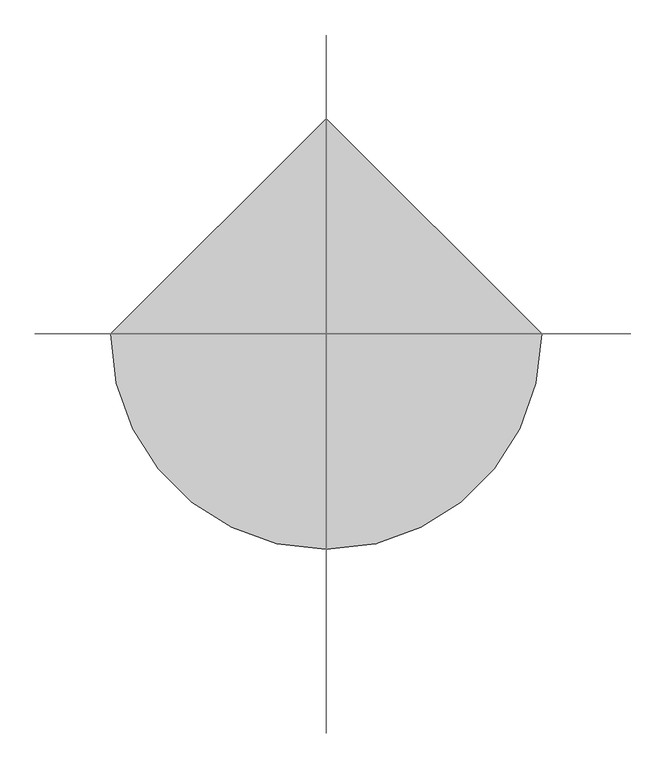
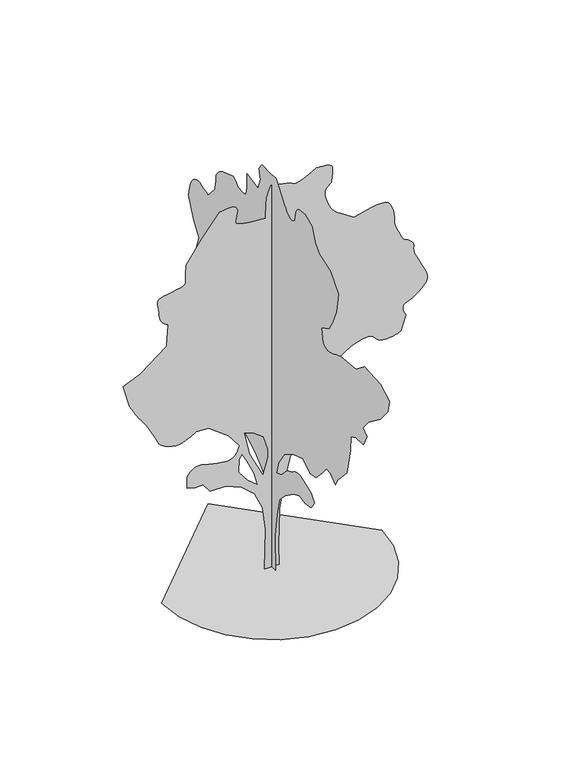
"""IFC4 building model written with IfcOpenShell, lengths in millimetres: proxy geometry, japanese flowering cherry 26172 : japanese flowering cherry 26172."""

from ifc_helpers import new_model, si_unit, origin, place, context, project, spatial, triangles, source, transform, mapped, element, save


def entourage_e499737d(model_context):
    return source(origin(), model_context, "Body", "Tessellation", [
        triangles([(-0.0028028, 75.7657196, 0.0059537), (-0.0028028, -73.2478183, 0.0059537), (-0.0028028, -59.7012251, 399.6312029), (-0.0028028, -100.3410047, 663.7914597), (-0.0028028, -147.7544623, 866.9916292), (-0.0028028, -256.1287339, 982.1375078), (-0.0028028, -418.6863261, 1097.2859299), (-0.0028028, -527.0605977, 1144.6976435), (-0.0028028, -635.434833, 1124.3775902), (-0.0028028, -750.5807842, 1144.6976435), (-0.0028028, -811.5407988, 1232.7519344), (-0.0028028, -750.5807842, 1314.0320023), (-0.0028028, -533.8347845, 1388.5377743), (-0.0028028, -514.9955638, 1387.0189716), (-0.0028028, -496.3341665, 1385.0834793), (-0.0028028, -478.0283798, 1382.3173691), (-0.0028028, -460.2559908, 1378.3091835), (-0.0028028, -443.1947865, 1372.6425236), (-0.0028028, -427.0200471, 1364.9005543), (-0.0028028, -411.9146828, 1354.6719635), (-0.0028028, -396.8067387, 1343.65345), (-0.0028028, -380.6345427, 1333.6991158), (-0.0028028, -363.5733384, 1324.6364422), (-0.0028028, -345.8009494, 1316.2824463), (-0.0028028, -327.4951627, 1308.4643188), (-0.0028028, -308.8337654, 1300.9992222), (-0.0028028, -289.994581, 1293.7118763), (-0.0028028, -188.3942419, 1185.3376774), (-0.0028028, -86.7944115, 1144.6976435), (-0.0028028, -127.4344454, 1286.9377258), (-0.0028028, -242.580869, 1456.2720119), (-0.0028028, -405.140496, 1557.8722057), (-0.0028028, -594.794799, 1618.8321476), (-0.0028028, -730.2607309, 1530.7779293), (-0.0028028, -838.6350025, 1544.3263756), (-0.0028028, -953.7809538, 1666.2439339), (-0.0028028, -1041.8351721, 1774.6181328), (-0.0028028, -1123.1126965, 1767.8439823), (-0.0028028, -1211.1669147, 1686.5663853), (-0.0028028, -1265.3528515, 1781.3922832), (-0.0028028, -1326.3127934, 1849.1240501), (-0.0028028, -1434.6871376, 1964.2723995), (-0.0028028, -1502.4187592, 2269.0726902), (-0.0028028, -1509.193055, 2431.6328259), (-0.0028028, -1604.0214237, 2472.2703163), (-0.0028028, -1753.0332584, 2485.8186172), (-0.0028028, -1813.9932003, 2614.5002975), (-0.0028028, -1739.4874283, 2675.4602394), (-0.0028028, -1841.0874767, 2797.3804138), (-0.0028028, -2071.3792339, 2973.5042564), (-0.0028028, -2220.3935394, 3149.6025192), (-0.0028028, -2247.4851997, 3291.8426743), (-0.0028028, -2078.1535297, 3386.6610146), (-0.0028028, -1766.5790886, 3400.2244308), (-0.0028028, -1610.7931034, 3278.3045471), (-0.0028028, -1312.7669632, 3244.4208595), (-0.0028028, -1272.2845505, 3228.5456657), (-0.0028028, -1232.7519344, 3213.2041603), (-0.0028028, -1195.1115721, 3198.9294502), (-0.0028028, -1160.3186377, 3186.2546425), (-0.0028028, -1129.3153702, 3175.7137161), (-0.0028028, -1103.0517843, 3167.8397781), (-0.0028028, -1082.4726625, 3163.1406464), (-0.0028028, -1064.0500225, 3162.8865921), (-0.0028028, -1044.5580437, 3166.9000099), (-0.0028028, -1025.4242552, 3173.6309944), (-0.0028028, -1008.065867, 3181.5558014), (-0.0028028, -993.907865, 3189.1248161), (-0.0028028, -984.3701477, 3194.789296), (-0.0028028, -980.8726141, 3197.024334), (-0.0028028, -947.0067307, 3359.5844696), (-0.0028028, -1089.2468857, 3434.0828293), (-0.0028028, -1156.9810507, 3542.4645859), (-0.0028028, -1231.4868954, 3718.5628487), (-0.0028028, -1272.127002, 3942.0832169), (-0.0028028, -1116.3410168, 4118.1814796), (-0.0028028, -913.1409199, 4192.7051285), (-0.0028028, -831.8608521, 4267.2034882), (-0.0028028, -770.9007648, 4429.7636238), (-0.0028028, -628.6606825, 4483.9417122), (-0.0028028, -605.4958537, 4483.8402649), (-0.0028028, -582.6891789, 4483.1542603), (-0.0028028, -560.5911455, 4481.2747238), (-0.0028028, -539.5599438, 4477.6426781), (-0.0028028, -519.9511116, 4471.5974075), (-0.0028028, -502.1202959, 4462.6310944), (-0.0028028, -486.4205638, 4450.0836044), (-0.0028028, -473.6824242, 4434.3863068), (-0.0028028, -464.1447433, 4416.5554184), (-0.0028028, -457.2740144, 4396.9467316), (-0.0028028, -452.5343691, 4375.9154572), (-0.0028028, -449.3949532, 4353.8173874), (-0.0028028, -447.3197528, 4331.0083145), (-0.0028028, -445.7805299, 4307.8434494), (-0.0028028, -434.0914178, 4294.9401672), (-0.0028028, -421.9248276, 4283.0531021), (-0.0028028, -408.8133096, 4273.1978897), (-0.0028028, -394.279422, 4266.3398781), (-0.0028028, -377.850701, 4263.5202827), (-0.0028028, -359.0495956, 4265.7303223), (-0.0028028, -337.4062583, 4273.9853416), (-0.0028028, -315.9610193, 4285.9741447), (-0.0028028, -297.7161846, 4298.6995308), (-0.0028028, -282.1358129, 4312.0091835), (-0.0028028, -268.6864885, 4325.8013649), (-0.0028028, -256.8373934, 4339.9237587), (-0.0028028, -246.0563473, 4354.3002068), (-0.0028028, -235.8074452, 4368.8033913), (-0.0028028, -140.9810386, 4497.5054192), (-0.0028028, -80.0209877, 4572.0037788), (-0.0028028, 21.579147, 4565.2219254), (-0.0028028, 184.1389784, 4572.0037788), (-0.0028028, 245.0987749, 4490.7235657), (-0.0028028, 218.0055885, 4375.5852448), (-0.0028028, 265.4200454, 4246.8835075), (-0.0028028, 475.3918765, 4287.5234688), (-0.0028028, 475.3918765, 4138.5014603), (-0.0028028, 476.9514107, 4115.4383331), (-0.0028028, 479.1637756, 4093.1623672), (-0.0028028, 482.6791134, 4072.5630432), (-0.0028028, 488.1502911, 4054.4781006), (-0.0028028, 496.2249435, 4039.6699928), (-0.0028028, 507.5609885, 4029.0273285), (-0.0028028, 522.8060609, 4023.3631393), (-0.0028028, 540.2228757, 4021.2551285), (-0.0028028, 557.6396542, 4020.5691238), (-0.0028028, 575.056469, 4021.0519432), (-0.0028028, 592.4732474, 4022.4995293), (-0.0028028, 609.8900259, 4024.6586998), (-0.0028028, 627.3093842, 4027.2748192), (-0.0028028, 644.726199, 4030.1449928), (-0.0028028, 660.7002239, 4045.9437378), (-0.0028028, 676.7352917, 4060.8791634), (-0.0028028, 692.8896835, 4074.0362091), (-0.0028028, 709.2193554, 4084.5265572), (-0.0028028, 725.7878208, 4091.4607269), (-0.0028028, 742.6534338, 4093.9498192), (-0.0028028, 759.8720776, 4091.1049347), (-0.0028028, 942.7522665, 4030.1449928), (-0.0028028, 968.7009007, 4012.6698967), (-0.0028028, 993.5827394, 3994.8390083), (-0.0028028, 1016.3309875, 3976.2971169), (-0.0028028, 1035.8813931, 3956.6881393), (-0.0028028, 1051.1646172, 3935.6568649), (-0.0028028, 1061.1163353, 3912.8477921), (-0.0028028, 1064.6722956, 3887.9048378), (-0.0028028, 1065.462291, 3862.3526184), (-0.0028028, 1067.6745832, 3837.8921928), (-0.0028028, 1071.0705969, 3814.3209572), (-0.0028028, 1075.4140091, 3791.4610153), (-0.0028028, 1080.4685698, 3769.1088913), (-0.0028028, 1085.9981741, 3747.1381393), (-0.0028028, 1091.7640285, 3725.3447021), (-0.0028028, 1220.4582081, 3583.1045471), (-0.0028028, 1259.5970982, 3600.2497215), (-0.0028028, 1298.4413841, 3615.8705704), (-0.0028028, 1336.691375, 3628.418351), (-0.0028028, 1374.0521759, 3636.343158), (-0.0028028, 1410.2294735, 3638.0956673), (-0.0028028, 1444.9259022, 3632.1521347), (-0.0028028, 1477.8442417, 3616.9629456), (-0.0028028, 1506.4193871, 3593.4931572), (-0.0028028, 1528.9517326, 3564.3086014), (-0.0028028, 1546.4471764, 3530.3996246), (-0.0028028, 1559.9143776, 3492.7059952), (-0.0028028, 1570.361269, 3452.1674812), (-0.0028028, 1578.7941845, 3409.7241417), (-0.0028028, 1586.218586, 3366.3410339), (-0.0028028, 1498.1643677, 3136.0643921), (-0.0028028, 1389.7926395, 2987.0423836), (-0.0028028, 1477.8442417, 2743.2023254), (-0.0028028, 1396.5641739, 2614.5002975), (-0.0028028, 1363.3893093, 2602.8164177), (-0.0028028, 1331.4588455, 2590.6497185), (-0.0028028, 1302.0151485, 2577.543251), (-0.0028028, 1276.3027645, 2563.0144867), (-0.0028028, 1255.5687103, 2546.5806061), (-0.0028028, 1241.0552067, 2527.7820442), (-0.0028028, 1234.0040382, 2506.1385979), (-0.0028028, 1231.6953129, 2483.1135498), (-0.0028028, 1230.4506214, 2460.4416779), (-0.0028028, 1230.0949745, 2438.0692062), (-0.0028028, 1230.4506214, 2415.9330574), (-0.0028028, 1231.339666, 2393.9721886), (-0.0028028, 1232.5842121, 2372.13326), (-0.0028028, 1234.0040382, 2350.3502872), (-0.0028028, 1206.9124506, 2241.9785591), (-0.0028028, 1017.2581112, 2262.2985397), (-0.0028028, 1001.4999161, 2230.5052769), (-0.0028028, 986.9863398, 2199.5401611), (-0.0028028, 974.9594576, 2170.2361359), (-0.0028028, 966.6663591, 2143.4188774), (-0.0028028, 963.3491198, 2119.9211838), (-0.0028028, 966.2523582, 2100.5664059), (-0.0028028, 976.6180773, 2086.1925739), (-0.0028028, 993.4227201, 2074.2646683), (-0.0028028, 1014.0196461, 2062.1005852), (-0.0028028, 1037.2225176, 2050.292149), (-0.0028028, 1061.8478313, 2039.431184), (-0.0028028, 1086.7093952, 2030.1093693), (-0.0028028, 1110.6234879, 2022.9211452), (-0.0028028, 1132.4039898, 2018.4583363), (-0.0028028, 1152.1322187, 2014.567004), (-0.0028028, 1170.7936523, 2008.9003441), (-0.0028028, 1188.5660414, 2001.7526699), (-0.0028028, 1205.6272093, 1993.4190216), (-0.0028028, 1222.157523, 1984.1961834), (-0.0028028, 1238.3297916, 1974.3816662), (-0.0028028, 1254.3241642, 1964.2723995), (-0.0028028, 1410.1126202, 2045.5524673), (-0.0028028, 1454.8979679, 2056.9850544), (-0.0028028, 1498.4412403, 2067.3533169), (-0.0028028, 1539.4952751, 2075.5879887), (-0.0028028, 1576.817997, 2080.6222744), (-0.0028028, 1609.1650051, 2081.3919949), (-0.0028028, 1635.2914627, 2076.8326801), (-0.0028028, 1653.9502075, 2065.8725933), (-0.0028028, 1666.2946575, 2049.9747265), (-0.0028028, 1674.7249569, 2031.5900928), (-0.0028028, 1679.8989143, 2011.1329113), (-0.0028028, 1682.4669262, 1989.0146393), (-0.0028028, 1683.0789528, 1965.6542919), (-0.0028028, 1682.3881519, 1941.4631813), (-0.0028028, 1681.0444839, 1916.8582878), (-0.0028028, 1657.7627655, 1892.3904499), (-0.0028028, 1634.1255455, 1869.1697742), (-0.0028028, 1609.7770317, 1848.4331039), (-0.0028028, 1584.3618679, 1831.4303627), (-0.0028028, 1557.5241165, 1819.4059513), (-0.0028028, 1528.9110374, 1813.5996197), (-0.0028028, 1498.1643677, 1815.2582394), (-0.0028028, 1465.6015297, 1822.4057682), (-0.0028028, 1432.5637207, 1830.9782101), (-0.0028028, 1400.2370602, 1839.0732101), (-0.0028028, 1369.8078129, 1844.8009129), (-0.0028028, 1342.4571568, 1846.2614342), (-0.0028028, 1319.3735367, 1841.5624477), (-0.0028028, 1301.7382759, 1828.8040695), (-0.0028028, 1288.4084209, 1812.3752758), (-0.0028028, 1277.2120113, 1797.7219551), (-0.0028028, 1267.7912201, 1784.5521194), (-0.0028028, 1259.7953419, 1772.5657871), (-0.0028028, 1252.8636429, 1761.4660286), (-0.0028028, 1246.6430923, 1750.9605652), (-0.0028028, 1240.778334, 1740.752322), (-0.0028028, 1263.8618088, 1737.6916077), (-0.0028028, 1286.1172817, 1733.6834221), (-0.0028028, 1306.714135, 1727.7779686), (-0.0028028, 1324.821896, 1719.0302467), (-0.0028028, 1339.6122723, 1706.4901691), (-0.0028028, 1350.2574074, 1689.2105553), (-0.0028028, 1355.9242126, 1666.2439339), (-0.0028028, 1358.2355541, 1639.3300243), (-0.0028028, 1359.4802456, 1610.9912018), (-0.0028028, 1359.8357471, 1581.4687305), (-0.0028028, 1359.4802456, 1550.9989334), (-0.0028028, 1358.591201, 1519.8178425), (-0.0028028, 1357.3466549, 1488.1643967), (-0.0028028, 1355.9242126, 1456.2720119), (-0.0028028, 1321.1312782, 1430.3436527), (-0.0028028, 1286.5720505, 1405.5990875), (-0.0028028, 1252.4876484, 1383.2266159), (-0.0028028, 1219.1146128, 1364.4078518), (-0.0028028, 1186.6915192, 1350.328624), (-0.0028028, 1155.4494581, 1342.1725811), (-0.0028028, 1125.6323828, 1341.1261333), (-0.0028028, 1095.812764, 1344.8167511), (-0.0028028, 1064.5732464, 1349.9322819), (-0.0028028, 1032.1476093, 1356.2316067), (-0.0028028, 998.774501, 1363.478112), (-0.0028028, 964.6902443, 1371.4385273), (-0.0028028, 930.1334873, 1379.8688267), (-0.0028028, 895.3380095, 1388.5377743), (-0.0028028, 692.1378399, 1341.1261333), (-0.0028028, 455.0718596, 1219.2061043), (-0.0028028, 319.6059277, 1144.6976435), (-0.0028028, 163.8189614, 1016.005862), (-0.0028028, 68.9922959, 819.5799156), (-0.0028028, 41.8991095, 541.8713216), (-0.0028028, 68.9922959, 264.1652892), (80.2102203, 0.0002552, 0.0), (-82.349661, 0.0002552, 0.0), (-68.8030678, 0.0002233, 460.5862032), (-102.6694236, 0.000202, 724.7463873), (-190.7229152, 0.0001914, 914.3981833), (-332.9637969, 0.0001914, 1043.0925081), (-509.0697627, 0.0001807, 1117.5983528), (-678.4015417, 0.0001807, 1117.5983528), (-759.684153, 0.0001807, 1219.1984013), (-847.7358278, 0.0001807, 1219.1984013), (-935.7901188, 0.0001807, 1239.5183819), (-935.7901188, 0.0001701, 1368.2127068), (-918.2539072, 0.0001701, 1391.2175526), (-900.0065472, 0.0001701, 1412.9192802), (-880.3392883, 0.0001595, 1432.0150623), (-858.5384388, 0.0001595, 1447.2017807), (-833.8928501, 0.0001595, 1457.1737011), (-805.6936993, 0.0001595, 1460.6307575), (-773.2299831, 0.0001595, 1456.266925), (-734.6829174, 0.0001595, 1446.5108345), (-690.4487715, 0.0001595, 1435.4516258), (-643.1335636, 0.0001701, 1424.2757092), (-595.3460009, 0.0001701, 1414.1639717), (-549.689449, 0.0001701, 1406.3051491), (-508.7725788, 0.0001701, 1401.8804192), (-475.2013721, 0.0001701, 1402.0785175), (-448.544024, 0.0001701, 1408.1415195), (-426.1513865, 0.0001701, 1419.8916744), (-407.3122021, 0.0001595, 1436.3813656), (-391.3152497, 0.0001595, 1456.660651), (-377.4544679, 0.0001595, 1479.7848209), (-365.0135485, 0.0001595, 1504.8039333), (-353.2838139, 0.0001595, 1530.7728424), (-475.2013721, 0.0001488, 1693.3329781), (-698.7215223, 0.0001382, 1855.8931137), (-834.1899977, 0.0001382, 1862.6647934), (-856.0492739, 0.0001382, 1849.6320133), (-878.4419477, 0.0001382, 1836.7771294), (-901.9038877, 0.0001382, 1824.277747), (-926.9610065, 0.0001382, 1812.3092915), (-954.1543322, 0.0001382, 1801.0544552), (-984.01203, 0.0001382, 1790.6861927), (-1017.0701866, 0.0001488, 1781.3847256), (-1055.1015862, 0.0001488, 1778.1664627), (-1097.4002398, 0.0001488, 1784.6638859), (-1140.7656887, 0.0001382, 1798.9792912), (-1182.0000904, 0.0001382, 1819.2206429), (-1217.9005154, 0.0001382, 1843.490237), (-1245.2690483, 0.0001382, 1869.8935673), (-1260.907774, 0.0001382, 1896.5332203), (-1274.5551968, 0.0001382, 1929.7461639), (-1296.2570698, 0.0001276, 1973.9803825), (-1323.2903034, 0.0001276, 2024.4959038), (-1352.9320988, 0.0001276, 2076.5482498), (-1382.45457, 0.0001276, 2125.4025352), (-1409.1321568, 0.0001169, 2166.3195145), (-1430.2420601, 0.0001169, 2194.5592152), (-1448.055217, 0.0001169, 2217.0508656), (-1466.5769062, 0.0001169, 2243.4541958), (-1485.6928905, 0.0001169, 2273.113868), (-1505.2813751, 0.0001169, 2305.3794857), (-1525.2255066, 0.0001063, 2339.6035595), (-1545.4082863, 0.0001063, 2375.12799), (-1565.7080647, 0.0001063, 2411.3051422), (-1640.2164528, 9.57e-05, 2668.7039658), (-1443.7878902, 8.51e-05, 2749.9838882), (-1159.310269, 7.44e-05, 2973.5042564), (-1145.7618954, 5.32e-05, 3217.3190254), (-1165.9447477, 5.32e-05, 3231.9748169), (-1185.2970549, 5.32e-05, 3247.3163223), (-1202.9906696, 5.32e-05, 3264.0804153), (-1218.1951195, 5.32e-05, 3282.9780991), (-1230.0823299, 5.32e-05, 3304.7203766), (-1237.8242992, 5.32e-05, 3330.0188324), (-1240.5902641, 5.32e-05, 3359.5591805), (-1243.0389519, 4.25e-05, 3392.8330215), (-1248.5659401, 4.25e-05, 3427.5294502), (-1254.4511913, 4.25e-05, 3461.7686394), (-1257.9665291, 4.25e-05, 3493.6204742), (-1256.3865383, 4.25e-05, 3521.204837), (-1246.9860947, 4.25e-05, 3542.6169022), (-1227.0419632, 4.25e-05, 3556.002713), (-1192.1092844, 4.25e-05, 3564.4103394), (-1144.1438982, 3.19e-05, 3572.715937), (-1090.0164608, 3.19e-05, 3581.5808029), (-1036.6002445, 3.19e-05, 3591.7915169), (-990.7659056, 3.19e-05, 3603.9835052), (-959.3867163, 3.19e-05, 3618.9186401), (-949.3359489, 3.19e-05, 3637.2829262), (-951.449192, 3.19e-05, 3659.3809959), (-952.1400656, 3.19e-05, 3684.6794518), (-951.644747, 3.19e-05, 3712.6448959), (-950.2045732, 3.19e-05, 3742.718351), (-948.0532511, 2.13e-05, 3774.4175789), (-945.4268852, 2.13e-05, 3807.1836021), (-942.5617258, 2.13e-05, 3840.4830231), (-773.2299831, 1.06e-05, 4084.3233719), (-576.803964, -1.06e-05, 4328.16343), (-534.9980856, -1.06e-05, 4335.1231796), (-494.9117606, -1.06e-05, 4340.3809982), (-458.2595647, -1.06e-05, 4342.2096657), (-426.7635221, -1.06e-05, 4338.8569633), (-402.1382083, -1.06e-05, 4328.6459587), (-386.1031769, -1.06e-05, 4309.850013), (-380.3754742, 0.0, 4280.7416153), (-383.1999384, 0.0, 4247.9503029), (-389.6972889, 0.0, 4219.0450905), (-396.9057878, 0.0, 4193.848082), (-401.8613357, 0.0, 4172.0549355), (-401.6048106, 0.0, 4153.462175), (-393.1720041, 0.0, 4137.8410355), (-373.6038308, 0.0, 4124.9633331), (-343.9238837, 0.0, 4114.5238541), (-307.8431645, 0.0, 4106.2435455), (-266.4335192, 1.06e-05, 4099.7157463), (-220.7586908, 1.06e-05, 4094.6355331), (-171.883967, 1.06e-05, 4090.5971169), (-120.8766607, 1.06e-05, 4087.2697037), (-68.8030678, 1.06e-05, 4084.3233719), (-62.0293897, 0.0, 4267.2034882), (-60.4495079, -1.06e-05, 4293.1367889), (-56.0260951, -1.06e-05, 4318.689299), (-49.2331141, -1.06e-05, 4343.962175), (-40.544273, -1.06e-05, 4369.0065765), (-30.4335416, -1.06e-05, 4393.8733727), (-19.3751868, -1.06e-05, 4418.612851), (-7.8427643, -1.06e-05, 4443.3017509), (38.3857792, -1.06e-05, 4434.5642029), (83.3110485, -1.06e-05, 4425.7249168), (125.6295138, -1.06e-05, 4416.6571564), (164.0381523, -1.06e-05, 4407.2083145), (197.2334371, -1.06e-05, 4397.3022331), (223.9120957, -1.06e-05, 4386.7865959), (242.7705922, -1.06e-05, 4375.5599556), (267.3174405, -1.06e-05, 4372.2834114), (307.2640574, -1.06e-05, 4382.5194145), (355.6256767, -1.06e-05, 4401.5188362), (405.4097383, -1.06e-05, 4424.5566742), (449.6235366, -1.06e-05, 4446.8576385), (481.2770551, -2.13e-05, 4463.7234695), (493.3827115, -2.13e-05, 4470.4035851), (503.1388384, -2.13e-05, 4470.6067703), (528.2975498, -2.13e-05, 4470.3274269), (562.6967946, -2.13e-05, 4468.2699944), (600.177065, -2.13e-05, 4463.1392029), (634.5763098, -1.06e-05, 4453.6142029), (659.7350212, -1.06e-05, 4438.3994339), (669.4911844, -1.06e-05, 4416.1999168), (669.0949877, -1.06e-05, 4390.4698013), (667.9900406, -1.06e-05, 4365.4506889), (666.2907984, -1.06e-05, 4341.0411324), (664.1190559, -1.06e-05, 4317.089106), (661.5918119, -1.06e-05, 4293.4922905), (658.8257017, 0.0, 4270.1245308), (655.9428108, 0.0, 4246.8835075), (638.6835445, 0.0, 4233.6753021), (622.3741476, 0.0, 4219.7308044), (607.9571134, 0.0, 4204.2114029), (596.3848546, 0.0, 4186.4060944), (588.6048426, 0.0, 4165.5271362), (585.5644395, 0.0, 4140.7876579), (588.2111166, 0.0, 4111.3996262), (595.5949319, 1.06e-05, 4078.8367882), (605.8235227, 1.06e-05, 4045.6643944), (618.4244614, 1.06e-05, 4012.9492401), (632.9176901, 1.06e-05, 3981.7834099), (648.8333611, 1.06e-05, 3953.233699), (665.698974, 1.06e-05, 3928.3416138), (683.0370146, 2.13e-05, 3908.1995293), (703.4154945, 2.13e-05, 3889.8099541), (729.1278786, 2.13e-05, 3869.6170006), (759.2802532, 2.13e-05, 3847.9505905), (792.9912043, 2.13e-05, 3825.1159378), (829.3639841, 2.13e-05, 3801.3670967), (867.5148531, 2.13e-05, 3777.0592781), (906.5572374, 2.13e-05, 3752.4212471), (974.48703, 2.13e-05, 3771.0140076), (1040.6997763, 2.13e-05, 3787.8795479), (1103.475959, 2.13e-05, 3801.2909386), (1161.1010027, 2.13e-05, 3809.5712471), (1211.8502306, 2.13e-05, 3810.9682549), (1254.0116833, 2.13e-05, 3803.7800308), (1285.8633728, 2.13e-05, 3786.2793549), (1308.8096466, 2.13e-05, 3757.831382), (1325.9495888, 3.19e-05, 3721.2045479), (1338.1136719, 3.19e-05, 3679.8280037), (1346.1325138, 3.19e-05, 3637.155899), (1350.8315002, 3.19e-05, 3596.6173851), (1353.0438652, 4.25e-05, 3561.641613), (1353.5976105, 4.25e-05, 3535.6827324), (1358.8503422, 4.25e-05, 3507.9969223), (1372.3961723, 4.25e-05, 3469.2870758), (1390.9178616, 4.25e-05, 3425.1418053), (1411.1006413, 5.32e-05, 3381.0982727), (1429.6249466, 5.32e-05, 3342.7442184), (1443.1707767, 5.32e-05, 3315.6423843), (1448.4235085, 5.32e-05, 3305.3808014), (1455.5126106, 5.32e-05, 3302.5614967), (1473.6202263, 5.32e-05, 3294.4079247), (1498.0094353, 5.32e-05, 3281.4031952), (1523.9376492, 5.32e-05, 3264.0042572), (1546.6656223, 5.32e-05, 3242.6936394), (1561.456144, 5.32e-05, 3217.9538704), (1563.5693871, 6.38e-05, 3190.2424805), (1560.9227463, 6.38e-05, 3161.8962456), (1563.9655838, 6.38e-05, 3134.3880409), (1571.7456322, 6.38e-05, 3106.8795456), (1583.3178909, 6.38e-05, 3078.5585999), (1597.7324181, 6.38e-05, 3048.5613029), (1614.0443584, 7.44e-05, 3016.0746231), (1631.3036247, 7.44e-05, 2980.2605301), (1651.0114334, 7.44e-05, 2941.4239471), (1672.8529781, 7.44e-05, 2900.911013), (1693.1526112, 7.44e-05, 2859.5850471), (1708.2377369, 8.51e-05, 2818.2593719), (1714.4404106, 8.51e-05, 2777.7461472), (1708.0801884, 8.51e-05, 2738.9095642), (1685.4894161, 8.51e-05, 2702.5620735), (1655.0603142, 9.57e-05, 2670.8884254), (1626.9983643, 9.57e-05, 2644.9042557), (1600.3587112, 9.57e-05, 2623.6442162), (1574.1941746, 9.57e-05, 2606.1944092), (1547.5546669, 9.57e-05, 2591.5894867), (1519.4951878, 9.57e-05, 2578.8641006), (1489.0634697, 9.57e-05, 2567.103772), (1463.2545799, 9.57e-05, 2553.5147758), (1448.4615875, 9.57e-05, 2536.3646599), (1442.8532089, 9.57e-05, 2516.2632706), (1444.5930737, 0.0001063, 2493.7893517), (1451.8397243, 0.0001063, 2469.5399597), (1462.7592613, 0.0001063, 2444.1069191), (1475.5176395, 0.0001063, 2418.079438), (1421.329232, 0.0001169, 2248.7450066), (1402.2741451, 0.0001169, 2240.1167542), (1382.0913654, 0.0001169, 2231.9607113), (1359.6579964, 0.0001169, 2224.752285), (1333.8491066, 0.0001169, 2218.9661556), (1303.5367126, 0.0001169, 2215.0772942), (1267.5955925, 0.0001169, 2213.5558754), (1224.9032856, 0.0001169, 2214.8791958), (1186.5543182, 0.0001169, 2223.6651421), (1160.2907324, 0.0001169, 2241.2216286), (1139.9504042, 0.0001169, 2263.0426804), (1119.3738258, 0.0001169, 2284.6250839), (1092.3990189, 0.0001169, 2301.470422), (1052.8638594, 0.0001169, 2309.0727196), (994.6089123, 0.0001169, 2302.9309433), (927.2531399, 0.0001169, 2283.7970821), (865.4625074, 0.0001169, 2256.8426228), (810.6645441, 0.0001169, 2224.1985397), (764.2764599, 0.0001169, 2188.0035107), (727.7258566, 0.0001169, 2150.3835686), (702.4274008, 0.0001276, 2113.4772457), (689.8112377, 0.0001276, 2079.4133366), (689.5343651, 0.0001276, 2049.0602474), (699.2092106, 0.0001276, 2021.5520428), (717.179698, 0.0001276, 1996.4136063), (741.7847368, 0.0001276, 1973.172583), (771.3655621, 0.0001382, 1951.3515312), (804.2662428, 0.0001382, 1930.4778053), (838.8229998, 0.0001382, 1910.0790504), (858.9855045, 0.0001382, 1896.9268009), (878.2006107, 0.0001382, 1883.2412991), (895.5183764, 0.0001382, 1868.4914726), (909.9938009, 0.0001382, 1852.1415985), (920.6770878, 0.0001382, 1833.6579884), (926.620693, 0.0001382, 1812.5073898), (926.8772181, 0.0001382, 1788.158876), (924.1721506, 0.0001488, 1758.4790016), (921.8225847, 0.0001488, 1722.4008259), (919.7677683, 0.0001488, 1680.9911442), (917.9516727, 0.0001488, 1635.3142811), (916.3107845, 0.0001595, 1586.4395027), (914.7919092, 0.0001595, 1535.4337498), (913.3288445, 0.0001595, 1483.3585854), (878.4571358, 0.0001595, 1457.529348), (843.3467062, 0.0001595, 1433.4780544), (807.7613056, 0.0001701, 1412.980323), (771.4646839, 0.0001701, 1397.8139523), (734.2231344, 0.0001701, 1389.7570312), (695.792922, 0.0001701, 1390.585033), (655.9428108, 0.0001701, 1402.0785175), (615.8971447, 0.0001701, 1417.3236626), (576.9157305, 0.0001701, 1428.6597439), (538.820781, 0.0001595, 1436.7368671), (501.4395962, 0.0001595, 1442.205574), (464.5917727, 0.0001595, 1445.7209118), (428.0995597, 0.0001595, 1447.9332767), (391.7826267, 0.0001595, 1449.4927746), (276.6366936, 0.0001701, 1374.9868572), (202.1305764, 0.0001807, 1205.6525711), (127.6236689, 0.0001914, 921.1724064), (86.9838894, 0.0002126, 643.4663195), (73.4370464, 0.0002339, 237.0665254), (-95.8962542, 8.51e-05, 1097.2783722), (-41.7096271, 7.44e-05, 1286.9326389), (-41.7096271, 6.38e-05, 1381.7585369), (-89.122576, 5.32e-05, 1544.3186726), (-211.0424234, 5.32e-05, 1632.3728909), (-305.8695931, 5.32e-05, 1666.238847), (-244.9095423, 6.38e-05, 1395.3069832), (-156.8557963, 6.38e-05, 1009.2266247), (-197.4958302, 6.38e-05, 1158.2383867), (-272.003746, 5.32e-05, 1320.7984497), (-326.1896101, 4.25e-05, 1422.3986435), (-360.0554572, 4.25e-05, 1374.9868572), (-366.829644, 5.32e-05, 1225.9725517), (-265.2295592, 6.38e-05, 1097.2783722), (-1212.9170259, 0.0, 0.0045929), (-1180.85205, -277.9194097, 0.0045929), (-1089.5287725, -533.1464181, 0.0045929), (-946.2625174, -758.3633034, 0.0045929), (-758.3633034, -946.2625174, 0.0045929), (-533.1464181, -1089.5287725, 0.0045929), (-277.9194097, -1180.85205, 0.0045929), (5.3e-05, -1212.9170259, 0.0045929), (277.9194097, -1180.85205, 0.0045929), (533.1464181, -1089.5287725, 0.0045929), (758.3633034, -946.2625174, 0.0045929), (946.2625174, -758.3633034, 0.0045929), (1089.5287725, -533.1464181, 0.0045929), (1180.85205, -277.9194097, 0.0045929), (1212.9170259, 0.0001063, 0.0045929), (-0.0001591, 1212.9170259, 0.0045929)], [[38, 39, 40], [115, 116, 117], [1, 2, 3], [280, 1, 3], [279, 280, 3], [279, 3, 4], [278, 279, 4], [278, 4, 5], [186, 187, 188], [277, 278, 5], [46, 47, 48], [45, 46, 48], [277, 5, 6], [185, 186, 188], [10, 11, 12], [9, 10, 12], [9, 12, 13], [8, 9, 13], [8, 13, 14], [8, 14, 15], [8, 15, 16], [8, 16, 17], [8, 17, 18], [8, 18, 19], [8, 19, 20], [8, 20, 21], [7, 8, 21], [7, 21, 22], [7, 22, 23], [7, 23, 24], [7, 24, 25], [7, 25, 26], [6, 7, 26], [6, 26, 27], [6, 27, 28], [277, 6, 28], [277, 28, 29], [51, 52, 53], [50, 51, 53], [50, 53, 54], [50, 54, 55], [49, 50, 55], [49, 55, 56], [48, 49, 56], [48, 56, 57], [45, 48, 57], [44, 45, 57], [44, 57, 58], [44, 58, 59], [44, 59, 60], [44, 60, 61], [44, 61, 62], [44, 62, 63], [276, 277, 29], [276, 29, 30], [184, 185, 188], [183, 184, 188], [44, 63, 64], [115, 117, 118], [111, 112, 113], [111, 113, 114], [182, 183, 188], [109, 110, 111], [109, 111, 114], [108, 109, 114], [108, 114, 115], [107, 108, 115], [106, 107, 115], [105, 106, 115], [104, 105, 115], [115, 118, 119], [170, 171, 172], [170, 172, 173], [170, 173, 174], [170, 174, 175], [74, 75, 76], [74, 76, 77], [73, 74, 77], [72, 73, 77], [71, 72, 77], [258, 259, 260], [181, 182, 188], [78, 79, 80], [170, 175, 176], [103, 104, 115], [78, 80, 81], [44, 64, 65], [275, 276, 30], [275, 30, 31], [274, 275, 31], [78, 81, 82], [78, 82, 83], [78, 83, 84], [78, 84, 85], [78, 85, 86], [78, 86, 87], [78, 87, 88], [78, 88, 89], [78, 89, 90], [78, 90, 91], [78, 91, 92], [78, 92, 93], [78, 93, 94], [78, 94, 95], [78, 95, 96], [71, 77, 78], [71, 78, 96], [71, 96, 97], [71, 97, 98], [71, 98, 99], [71, 99, 100], [115, 119, 120], [180, 181, 188], [38, 40, 41], [223, 224, 225], [33, 34, 35], [33, 35, 36], [33, 36, 37], [102, 103, 115], [179, 180, 188], [44, 65, 66], [170, 176, 177], [71, 100, 101], [43, 44, 66], [42, 43, 66], [41, 42, 66], [38, 41, 66], [37, 38, 66], [33, 37, 66], [33, 66, 67], [33, 67, 68], [33, 68, 69], [33, 69, 70], [32, 33, 70], [31, 32, 70], [274, 31, 70], [273, 274, 70], [273, 70, 71], [273, 71, 101], [273, 101, 102], [273, 102, 115], [273, 115, 120], [273, 120, 121], [273, 121, 122], [273, 122, 123], [273, 123, 124], [273, 124, 125], [273, 125, 126], [273, 126, 127], [273, 127, 128], [273, 128, 129], [273, 129, 130], [273, 130, 131], [272, 273, 131], [271, 272, 131], [270, 271, 131], [269, 270, 131], [268, 269, 131], [268, 131, 132], [268, 132, 133], [268, 133, 134], [167, 168, 169], [257, 258, 260], [257, 260, 261], [256, 257, 261], [256, 261, 262], [255, 256, 262], [255, 262, 263], [254, 255, 263], [254, 263, 264], [254, 264, 265], [254, 265, 266], [254, 266, 267], [254, 267, 268], [253, 254, 268], [252, 253, 268], [251, 252, 268], [250, 251, 268], [249, 250, 268], [248, 249, 268], [247, 248, 268], [246, 247, 268], [245, 246, 268], [166, 167, 169], [165, 166, 169], [164, 165, 169], [163, 164, 169], [162, 163, 169], [161, 162, 169], [160, 161, 169], [159, 160, 169], [158, 159, 169], [157, 158, 169], [156, 157, 169], [155, 156, 169], [154, 155, 169], [154, 169, 170], [154, 170, 177], [153, 154, 177], [153, 177, 178], [153, 178, 179], [153, 179, 188], [222, 223, 225], [222, 225, 226], [221, 222, 226], [220, 221, 226], [219, 220, 226], [218, 219, 226], [217, 218, 226], [216, 217, 226], [215, 216, 226], [214, 215, 226], [213, 214, 226], [212, 213, 226], [212, 226, 227], [212, 227, 228], [212, 228, 229], [212, 229, 230], [212, 230, 231], [211, 212, 231], [211, 231, 232], [211, 232, 233], [210, 211, 233], [209, 210, 233], [209, 233, 234], [209, 234, 235], [209, 235, 236], [209, 236, 237], [209, 237, 238], [209, 238, 239], [209, 239, 240], [208, 209, 240], [208, 240, 241], [207, 208, 241], [206, 207, 241], [206, 241, 242], [205, 206, 242], [204, 205, 242], [204, 242, 243], [203, 204, 243], [202, 203, 243], [202, 243, 244], [201, 202, 244], [201, 244, 245], [201, 245, 268], [200, 201, 268], [199, 200, 268], [198, 199, 268], [197, 198, 268], [196, 197, 268], [195, 196, 268], [194, 195, 268], [153, 188, 189], [153, 189, 190], [152, 153, 190], [152, 190, 191], [151, 152, 191], [136, 137, 138], [135, 136, 138], [135, 138, 139], [134, 135, 139], [134, 139, 140], [134, 140, 141], [134, 141, 142], [134, 142, 143], [134, 143, 144], [134, 144, 145], [134, 145, 146], [134, 146, 147], [134, 147, 148], [134, 148, 149], [134, 149, 150], [134, 150, 151], [134, 151, 191], [134, 191, 192], [134, 192, 193], [268, 134, 193], [194, 268, 193], [583, 580, 581], [574, 281, 575], [580, 583, 584], [573, 574, 575], [583, 581, 575], [580, 584, 585], [572, 573, 575], [582, 583, 575], [582, 575, 281], [571, 572, 575], [571, 575, 576], [281, 282, 283], [570, 571, 576], [570, 576, 577], [344, 345, 346], [290, 291, 292], [406, 407, 408], [570, 577, 578], [290, 292, 293], [289, 290, 293], [289, 293, 294], [289, 294, 295], [289, 295, 296], [289, 296, 297], [289, 297, 298], [289, 298, 299], [289, 299, 300], [289, 300, 301], [289, 301, 302], [289, 302, 303], [288, 289, 303], [287, 288, 303], [287, 303, 304], [287, 304, 305], [287, 305, 306], [286, 287, 306], [286, 306, 307], [286, 307, 308], [286, 308, 309], [569, 570, 578], [554, 555, 556], [405, 406, 408], [343, 344, 346], [512, 513, 514], [511, 512, 514], [511, 514, 515], [511, 515, 516], [511, 516, 517], [510, 511, 517], [510, 517, 518], [510, 518, 519], [510, 519, 520], [510, 520, 521], [510, 521, 522], [510, 522, 523], [510, 523, 524], [509, 510, 524], [509, 524, 525], [508, 509, 525], [434, 435, 436], [342, 343, 346], [507, 508, 525], [507, 525, 526], [405, 408, 409], [404, 405, 409], [403, 404, 409], [403, 409, 410], [402, 403, 410], [401, 402, 410], [400, 401, 410], [400, 410, 411], [399, 400, 411], [399, 411, 412], [399, 412, 413], [399, 413, 414], [399, 414, 415], [377, 378, 379], [341, 342, 346], [341, 346, 347], [340, 341, 347], [339, 340, 347], [338, 339, 347], [337, 338, 347], [336, 337, 347], [335, 336, 347], [334, 335, 347], [333, 334, 347], [377, 379, 380], [377, 380, 381], [377, 381, 382], [377, 382, 383], [377, 383, 384], [377, 384, 385], [377, 385, 386], [377, 386, 387], [377, 387, 388], [377, 388, 389], [377, 389, 390], [377, 390, 391], [376, 377, 391], [376, 391, 392], [375, 376, 392], [374, 375, 392], [373, 374, 392], [372, 373, 392], [372, 392, 393], [371, 372, 393], [370, 371, 393], [369, 370, 393], [369, 393, 394], [369, 394, 395], [369, 395, 396], [332, 333, 347], [369, 396, 397], [426, 427, 428], [426, 428, 429], [425, 426, 429], [425, 429, 430], [424, 425, 430], [424, 430, 431], [423, 424, 431], [423, 431, 432], [422, 423, 432], [422, 432, 433], [421, 422, 433], [420, 421, 433], [419, 420, 433], [418, 419, 433], [418, 433, 434], [418, 434, 436], [418, 436, 437], [418, 437, 438], [418, 438, 439], [417, 418, 439], [417, 439, 440], [416, 417, 440], [416, 440, 441], [415, 416, 441], [399, 415, 441], [399, 441, 442], [399, 442, 443], [399, 443, 444], [399, 444, 445], [399, 445, 446], [399, 446, 447], [399, 447, 448], [399, 448, 449], [369, 397, 398], [331, 332, 347], [368, 369, 398], [360, 361, 362], [359, 360, 362], [359, 362, 363], [358, 359, 363], [358, 363, 364], [357, 358, 364], [357, 364, 365], [356, 357, 365], [355, 356, 365], [355, 365, 366], [354, 355, 366], [353, 354, 366], [352, 353, 366], [351, 352, 366], [350, 351, 366], [349, 350, 366], [348, 349, 366], [348, 366, 367], [348, 367, 368], [348, 368, 398], [347, 348, 398], [347, 398, 399], [347, 399, 449], [347, 449, 450], [347, 450, 451], [347, 451, 452], [331, 347, 452], [331, 452, 453], [331, 453, 454], [331, 454, 455], [331, 455, 456], [330, 331, 456], [329, 330, 456], [328, 329, 456], [327, 328, 456], [326, 327, 456], [325, 326, 456], [324, 325, 456], [323, 324, 456], [322, 323, 456], [321, 322, 456], [320, 321, 456], [319, 320, 456], [318, 319, 456], [317, 318, 456], [316, 317, 456], [315, 316, 456], [314, 315, 456], [314, 456, 457], [314, 457, 458], [314, 458, 459], [314, 459, 460], [314, 460, 461], [314, 461, 462], [314, 462, 463], [314, 463, 464], [314, 464, 465], [314, 465, 466], [314, 466, 467], [314, 467, 468], [314, 468, 469], [314, 469, 470], [314, 470, 471], [314, 471, 472], [314, 472, 473], [314, 473, 474], [314, 474, 475], [314, 475, 476], [314, 476, 477], [314, 477, 478], [314, 478, 479], [314, 479, 480], [314, 480, 481], [314, 481, 482], [314, 482, 483], [314, 483, 484], [314, 484, 485], [314, 485, 486], [314, 486, 487], [314, 487, 488], [314, 488, 489], [314, 489, 490], [314, 490, 491], [314, 491, 492], [314, 492, 493], [314, 493, 494], [314, 494, 495], [314, 495, 496], [314, 496, 497], [314, 497, 498], [314, 498, 499], [314, 499, 500], [314, 500, 501], [314, 501, 502], [580, 585, 586], [554, 556, 557], [553, 554, 557], [553, 557, 558], [553, 558, 559], [553, 559, 560], [553, 560, 561], [553, 561, 562], [553, 562, 563], [552, 553, 563], [552, 563, 564], [551, 552, 564], [550, 551, 564], [550, 564, 565], [549, 550, 565], [549, 565, 566], [548, 549, 566], [547, 548, 566], [546, 547, 566], [545, 546, 566], [544, 545, 566], [543, 544, 566], [542, 543, 566], [541, 542, 566], [540, 541, 566], [539, 540, 566], [538, 539, 566], [538, 566, 567], [537, 538, 567], [537, 567, 568], [537, 568, 569], [537, 569, 578], [536, 537, 578], [535, 536, 578], [535, 578, 579], [534, 535, 579], [534, 579, 580], [533, 534, 580], [532, 533, 580], [507, 526, 527], [506, 507, 527], [531, 532, 580], [506, 527, 528], [530, 531, 580], [281, 283, 284], [582, 281, 284], [582, 284, 285], [582, 285, 286], [588, 582, 286], [587, 588, 286], [587, 286, 309], [586, 587, 309], [586, 309, 310], [586, 310, 311], [586, 311, 312], [586, 312, 313], [580, 586, 313], [580, 313, 314], [530, 580, 314], [529, 530, 314], [502, 503, 504], [502, 504, 505], [314, 502, 505], [529, 314, 505], [529, 505, 506], [529, 506, 528], [603, 604, 589], [602, 603, 589], [602, 589, 590], [601, 602, 590], [601, 590, 591], [601, 591, 592], [600, 601, 592], [599, 600, 592], [599, 592, 593], [599, 593, 594], [599, 594, 595], [599, 595, 596], [599, 596, 597], [599, 597, 598]], closed=False),
    ])


if __name__ == "__main__":
    model = new_model("IFC4")
    model_context = context("Model", 3, world=origin())
    ifc_project = project(units=[si_unit("LENGTHUNIT", "METRE", prefix="MILLI")], contexts=[model_context])
    site = spatial("IfcSite", under=ifc_project)
    building = spatial("IfcBuilding", under=site)
    placement = place(None, origin())
    entourage_shape = entourage_e499737d(model_context)
    element("IfcBuildingElementProxy", 1, Name="japanese flowering cherry 26172 : japanese flowering cherry 26172", ObjectType="japanese flowering cherry 26172 : japanese flowering cherry 26172", at=placement, inside=building, context=model_context, shape_type="MappedRepresentation", body=[
        mapped(entourage_shape, transform((0.0, 0.0, 0.0), x_axis=(1.0, 0.0, 0.0), y_axis=(0.0, 1.0, 0.0), z_axis=(0.0, 0.0, 1.0))),
    ])
    save(model, "model.ifc")

# Revit data of these elements
# Type "japanese flowering cherry 26172 : japanese flowering cherry 26172"
#   built-in parameter 1005195 = "RPC-16-FXGW-2MQ0-PN7K-A000-ST1L-LVER-AU"
#   Height = 0
